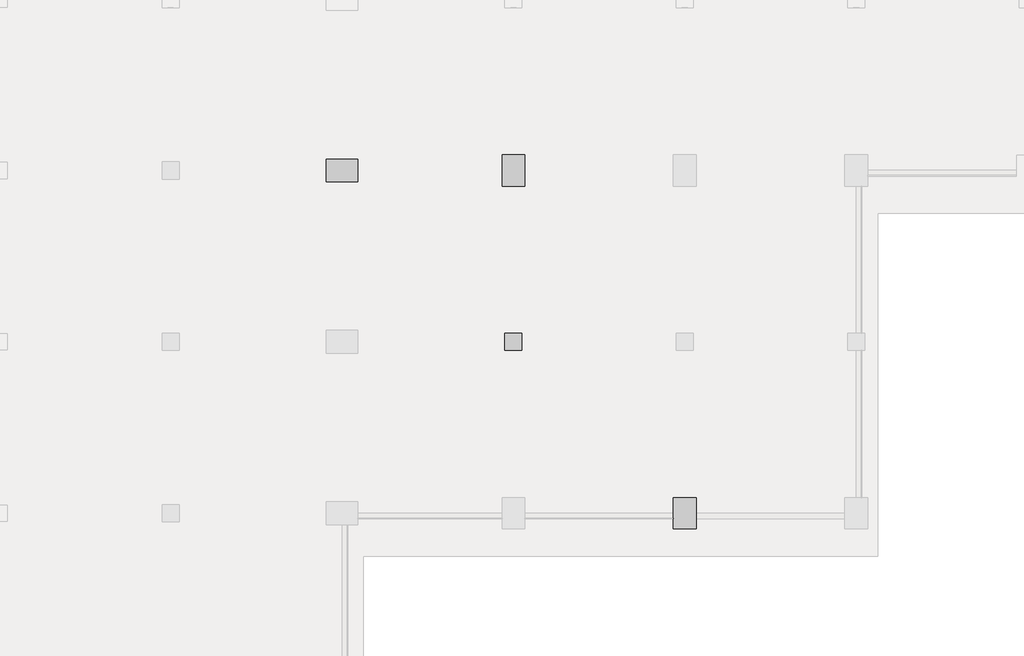
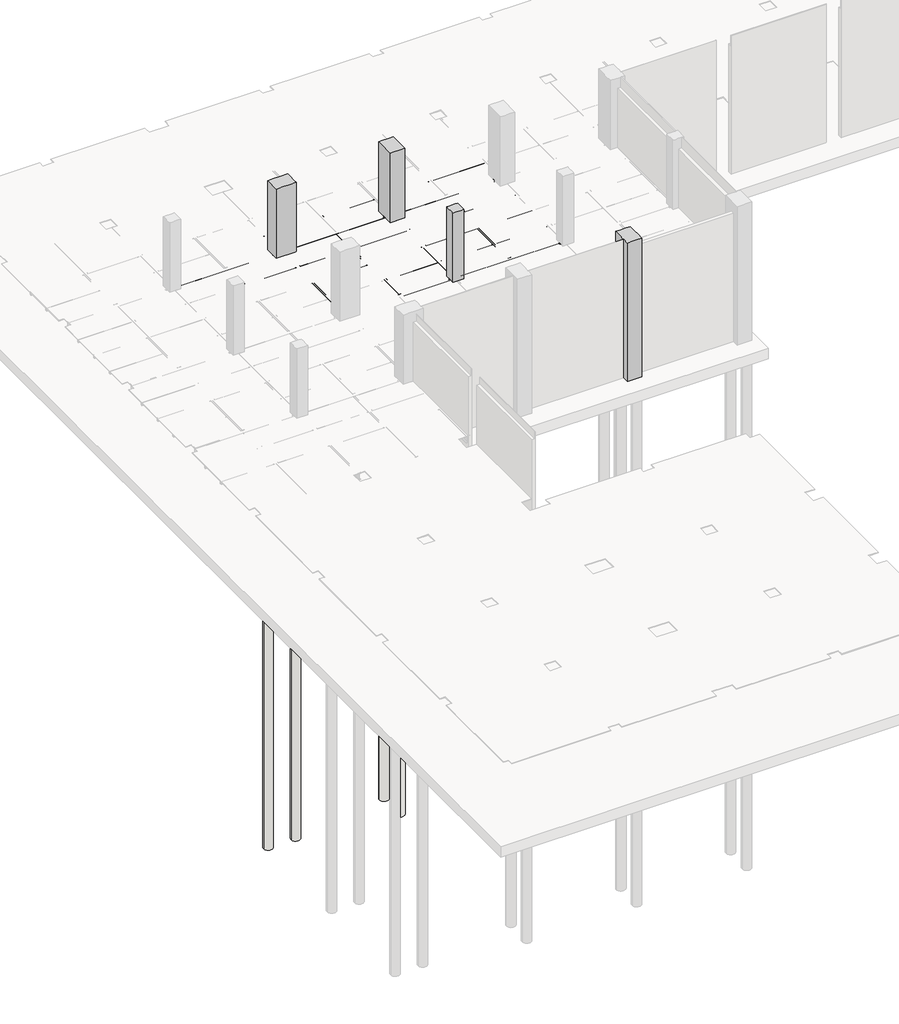
# Not in any storey, part 10 of 16: 28 beams, 6 slabs, 4 columns.
# Revit data of these elements (continued)
# Element 31 (IfcColumn, "RC_Column_Rectangular : H_SC_AR_S15_UG PED_Bit_600x600_BC1") (continued)
#   hec_material3 = none
#   hec_material2 = none
#   hec_material1 = none
#   Structural Material = 00_Concrete_Reinf. Conc.
#   Phase Created = New Construction
#   Materials on its faces: "00_Concrete_Reinf. Conc."
# Elements 33, 34, 35, 36, 37, 38 (IfcSlab, "PILE : H_SF_AR_S19_PHC Pile_Pre-boring_D500_L30")
#   Structural Material = none
#   Phase Created = New Construction
# Materials
#   "Steel, 45-345": class "Metal", colour RGB 189 187 185, transparency 0, Description = "Steel 345 MPa", Cost = 0
#   "00_Concrete_Reinf. Conc.": class "Concrete", colour RGB 176 176 176, transparency 0, Description = "Reinf. Conc.", Cost = 0, Image = Concrete.Cast-In-Place.Flat.Polished.Grey.jpg
